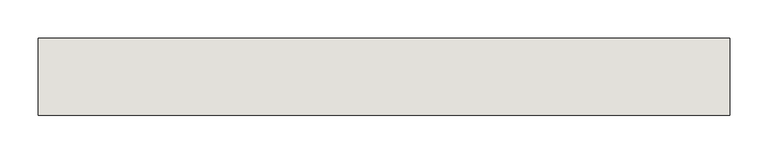
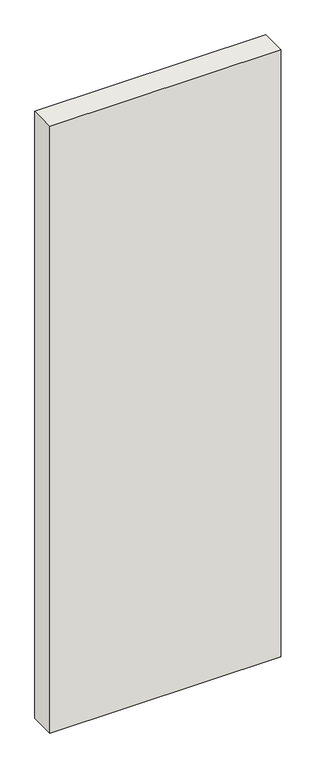
"""IFC4 building model written with IfcOpenShell, lengths in millimetres: wall geometry, Holzwand."""

from ifc_helpers import new_model, si_unit, origin, origin_with_axes, place, context, project, spatial, polyline, outline, extrude, source, transform, mapped, element, save


def wall_99b361a1(model_context):
    return source(origin(), model_context, "Body", "SweptSolid", [
        extrude(outline(polyline([(0.0, 100.0), (900.0, 100.0), (900.0, 0.0), (0.0, 0.0), (0.0, 100.0)])), origin_with_axes(), (0.0, 0.0, 1.0), 2500.0),
    ])


if __name__ == "__main__":
    model = new_model("IFC4")
    model_context = context("Model", 3, world=origin())
    ifc_project = project(units=[si_unit("LENGTHUNIT", "METRE", prefix="MILLI")], contexts=[model_context])
    site = spatial("IfcSite", under=ifc_project)
    building = spatial("IfcBuilding", under=site)
    placement = place(None, origin())
    wall_shape = wall_99b361a1(model_context)
    element("IfcWall", 1, ObjectType="Holzwand", at=placement, inside=building, context=model_context, shape_type="MappedRepresentation", body=[
        mapped(wall_shape, transform((0.0, 0.0, 0.0), x_axis=(1.0, 0.0, 0.0), y_axis=(0.0, 1.0, 0.0), z_axis=(0.0, 0.0, 1.0))),
    ])
    save(model, "model.ifc")

# Revit data of these elements
# Element 1 (IfcWall, "Holzwand")
#   Materials on its faces: "holzschalung"
# Materials
#   "holzschalung": class "Unassigned", colour RGB 128 128 128, transparency 0
